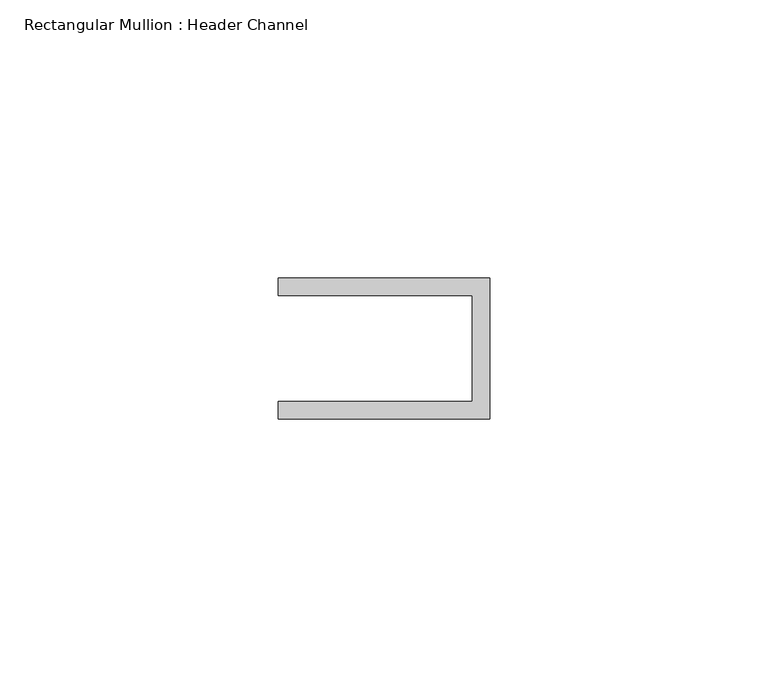
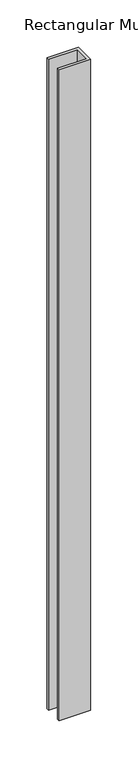
"""IFC4 building model written with IfcOpenShell, lengths in millimetres: member geometry, Rectangular Mullion : Header Channel."""

import ifcopenshell
import ifcopenshell.guid

model = None  # the IFC model being written
_history = None  # IfcOwnerHistory: only IFC2X3 demands one
_inside = {}  # id of a spatial element -> (the spatial element, [elements in it])
_under = {}  # id of a project, library or spatial element -> (it, [spatial elements below it])
_declared = {}  # id of a project -> (the project, [libraries it declares])
_typed = {}  # id of a type object -> (the type object, [elements of that type])
_made_of = {}  # id of a material, layer set ... -> (it, [elements and type objects made of it])


def new_model(schema):
    """Start an empty IFC model of exactly this schema.

    Asked for "IFC4X3", IfcOpenShell would pick the latest addendum, in which some entities
    have other attributes; the version numbers below select the first issue.
    IFC2X3 requires an IfcOwnerHistory on every rooted entity: one is made here for all.
    """
    global model, _history
    if schema == "IFC4X3":
        model = ifcopenshell.file(schema_version=(4, 3, 0, 0))
    else:
        model = ifcopenshell.file(schema=schema)
    _inside.clear()
    _under.clear()
    _declared.clear()
    _typed.clear()
    _made_of.clear()
    _history = None
    if model.schema == "IFC2X3":
        org = make("IfcOrganization", Name="unknown")
        user = make(
            "IfcPersonAndOrganization",
            ThePerson=make("IfcPerson", FamilyName="unknown"),
            TheOrganization=org,
        )
        app = make(
            "IfcApplication",
            ApplicationDeveloper=org,
            Version="unknown",
            ApplicationFullName="unknown",
            ApplicationIdentifier="unknown",
        )
        _history = make(
            "IfcOwnerHistory",
            OwningUser=user,
            OwningApplication=app,
            ChangeAction="ADDED",
            CreationDate=0,
        )
    return model


def make(cls, **values):
    """One entity of the class cls with the attributes given. An attribute that is None is left unset."""
    return model.create_entity(
        cls, **{name: value for name, value in values.items() if value is not None}
    )


def rooted(cls, **values):
    """An entity with a GlobalId (a new one), such as an element, a storey or a relation."""
    return make(cls, GlobalId=ifcopenshell.guid.new(), OwnerHistory=_history, **values)


def si_unit(unit_type, name, prefix=None):
    """IfcSIUnit, for example si_unit("LENGTHUNIT", "METRE", prefix="MILLI")."""
    return make("IfcSIUnit", UnitType=unit_type, Prefix=prefix, Name=name)


def assignment(units):
    """IfcUnitAssignment: the units of a project."""
    return None if units is None else make("IfcUnitAssignment", Units=units)


def point(xyz):
    """IfcCartesianPoint."""
    return None if xyz is None else make("IfcCartesianPoint", Coordinates=xyz)


def direction(xyz):
    """IfcDirection."""
    return None if xyz is None else make("IfcDirection", DirectionRatios=xyz)


def frame(location, z_axis=None, x_axis=None):
    """IfcAxis2Placement3D, a coordinate frame: its origin and axes. An axis left out is left unset."""
    return make(
        "IfcAxis2Placement3D",
        Location=point(location),
        Axis=direction(z_axis),
        RefDirection=direction(x_axis),
    )


def origin():
    """The frame at (0, 0, 0) with its axes left unset."""
    return frame((0.0, 0.0, 0.0))


def place(relative_to, where):
    """IfcLocalPlacement: puts the frame where relative to a parent placement (None: the world)."""
    return make(
        "IfcLocalPlacement", PlacementRelTo=relative_to, RelativePlacement=where
    )


def context(
    kind, dimensions, precision=None, world=None, true_north=None, identifier=None
):
    """IfcGeometricRepresentationContext, for example the 3D "Model" context."""
    return make(
        "IfcGeometricRepresentationContext",
        ContextIdentifier=identifier,
        ContextType=kind,
        CoordinateSpaceDimension=dimensions,
        Precision=precision,
        WorldCoordinateSystem=world,
        TrueNorth=true_north,
    )


def project(units=None, contexts=None):
    """IfcProject with its units and contexts."""
    return rooted(
        "IfcProject",
        Name="project",
        RepresentationContexts=contexts,
        UnitsInContext=assignment(units),
    )


def spatial(cls, under=None, at=None, **own):
    """A site, building, storey or space (cls), placed at a placement, below another one or the project."""
    s = rooted(cls, ObjectPlacement=at, **own)
    if under is not None:
        _under.setdefault(under.id(), (under, []))[1].append(s)
    return s


def polyline(points):
    """IfcPolyline through the points."""
    return make("IfcPolyline", Points=[point(p) for p in points])


def outline(outer, holes=None, kind="AREA"):
    """IfcArbitraryClosedProfileDef: a profile drawn as a closed curve; with holes, ...WithVoids."""
    if holes is None:
        return make("IfcArbitraryClosedProfileDef", ProfileType=kind, OuterCurve=outer)
    return make(
        "IfcArbitraryProfileDefWithVoids",
        ProfileType=kind,
        OuterCurve=outer,
        InnerCurves=holes,
    )


def extrude(swept, where, along, depth):
    """IfcExtrudedAreaSolid: the profile swept, set in the frame where, extruded along a direction by depth."""
    return make(
        "IfcExtrudedAreaSolid",
        SweptArea=swept,
        Position=where,
        ExtrudedDirection=direction(along),
        Depth=depth,
    )


def shape(context_of_items, identifier, shape_type, items):
    """IfcShapeRepresentation: the items that make up one representation, for example the "Body"."""
    return make(
        "IfcShapeRepresentation",
        ContextOfItems=context_of_items,
        RepresentationIdentifier=identifier,
        RepresentationType=shape_type,
        Items=items,
    )


def source(mapping_origin, context_of_items, identifier, shape_type, items):
    """IfcRepresentationMap: a shape defined once, which mapped items show again and again."""
    return make(
        "IfcRepresentationMap",
        MappingOrigin=mapping_origin,
        MappedRepresentation=shape(context_of_items, identifier, shape_type, items),
    )


def transform(
    local_origin,
    x_axis=None,
    y_axis=None,
    z_axis=None,
    scale=None,
    scale2=None,
    scale3=None,
    uniform=True,
):
    """IfcCartesianTransformationOperator3D, or its non-uniform kind. x_axis, y_axis, z_axis: its Axis1, 2, 3."""
    if uniform:
        return make(
            "IfcCartesianTransformationOperator3D",
            Axis1=direction(x_axis),
            Axis2=direction(y_axis),
            LocalOrigin=point(local_origin),
            Scale=scale,
            Axis3=direction(z_axis),
        )
    return make(
        "IfcCartesianTransformationOperator3DnonUniform",
        Axis1=direction(x_axis),
        Axis2=direction(y_axis),
        LocalOrigin=point(local_origin),
        Scale=scale,
        Axis3=direction(z_axis),
        Scale2=scale2,
        Scale3=scale3,
    )


def mapped(mapping_source, mapping_target):
    """IfcMappedItem: shows the shape of a source again, moved by a transform."""
    return make(
        "IfcMappedItem", MappingSource=mapping_source, MappingTarget=mapping_target
    )


def made_of(thing, what):
    """Note that an element or type object is made of a material, layer set ...; save() writes the relation."""
    if what is not None:
        _made_of.setdefault(what.id(), (what, []))[1].append(thing)
    return thing


def element(
    cls,
    number,
    at=None,
    inside=None,
    cuts=None,
    type_object=None,
    material=None,
    context=None,
    identifier="Body",
    shape_type=None,
    held_by="IfcProductDefinitionShape",
    body=None,
    shapes=None,
    **own,
):
    """One element of the class cls, such as IfcWall. Its Tag is "e" and its number.

    at: its placement. inside: the storey or other place that contains it. cuts: it is an
    opening in that element (IfcRelVoidsElement). A single representation is given by context,
    identifier, shape_type and body (its items); several are given by shapes. held_by: the class
    of the entity that holds the representations. save() writes the other relations.
    """
    e = rooted(cls, Tag="e%d" % number, ObjectPlacement=at, **own)
    if body is not None:
        shapes = [shape(context, identifier, shape_type, body)]
    if shapes is not None:
        e.Representation = make(held_by, Representations=shapes)
    if inside is not None:
        _inside.setdefault(inside.id(), (inside, []))[1].append(e)
    if cuts is not None:
        rooted(
            "IfcRelVoidsElement", RelatingBuildingElement=cuts, RelatedOpeningElement=e
        )
    if type_object is not None:
        _typed.setdefault(type_object.id(), (type_object, []))[1].append(e)
    return made_of(e, material)


def aggregate(whole, parts):
    """IfcRelAggregates: a whole, such as a stair, and the parts it consists of."""
    return rooted("IfcRelAggregates", RelatingObject=whole, RelatedObjects=parts)


def save(model, path):
    """Write the relations noted so far, then the file.

    IfcRelAggregates (storeys below a building ...), IfcRelContainedInSpatialStructure (elements
    in a storey), IfcRelDefinesByType, IfcRelAssociatesMaterial and IfcRelDeclares: one each for
    every whole, place, type object, material and project.
    """
    for whole, parts in _under.values():
        aggregate(whole, parts)
    for where, things in _inside.values():
        rooted(
            "IfcRelContainedInSpatialStructure",
            RelatedElements=things,
            RelatingStructure=where,
        )
    for kind, things in _typed.values():
        rooted("IfcRelDefinesByType", RelatedObjects=things, RelatingType=kind)
    for what, things in _made_of.values():
        rooted("IfcRelAssociatesMaterial", RelatedObjects=things, RelatingMaterial=what)
    for by, libraries in _declared.values():
        rooted("IfcRelDeclares", RelatingContext=by, RelatedDefinitions=libraries)
    model.write(path)


def rectangular_mullion_header_channel_0f02b38c(model_context):
    return source(origin(), model_context, "Body", "SweptSolid", [
        extrude(outline(polyline([(0.0, -12.7), (-38.1, -12.7), (-38.1, -9.525), (-3.175, -9.525), (-3.175, 9.525), (-38.1, 9.525), (-38.1, 12.7), (0.0, 12.7), (0.0, -12.7)])), frame((0.0, 0.0, -838.1999999), z_axis=(0.0, 0.0, 1.0), x_axis=(1.0, 0.0, 0.0)), (0.0, 0.0, 1.0), 838.1999999),
    ])


if __name__ == "__main__":
    model = new_model("IFC4")
    model_context = context("Model", 3, world=origin())
    ifc_project = project(units=[si_unit("LENGTHUNIT", "METRE", prefix="MILLI")], contexts=[model_context])
    site = spatial("IfcSite", under=ifc_project)
    building = spatial("IfcBuilding", under=site)
    placement = place(None, origin())
    rectangular_mullion_header_channel_shape = rectangular_mullion_header_channel_0f02b38c(model_context)
    element("IfcMember", 1, ObjectType="Rectangular Mullion : Header Channel", at=placement, inside=building, context=model_context, shape_type="MappedRepresentation", body=[
        mapped(rectangular_mullion_header_channel_shape, transform((0.0, 0.0, 0.0), x_axis=(1.0, 0.0, 0.0), y_axis=(0.0, 1.0, 0.0), z_axis=(0.0, 0.0, 1.0))),
    ])
    save(model, "model.ifc")

# Revit data of these elements
# Type "Rectangular Mullion : Header Channel"
#   built-in parameter 1007322 = 0.0833333 (stored number, unit not read)
#   built-in parameter 1007321 = -0.03125 (stored number, unit not read)
#   built-in parameter 1007320 = 0.0416667 (stored number, unit not read)
# Element 1 (IfcMember, "Rectangular Mullion : Header Channel")
#   Materials on its faces: "ALUM"
# Materials
#   "ALUM": class "Generic", colour RGB 157 157 157, transparency 0, Cost = 0
